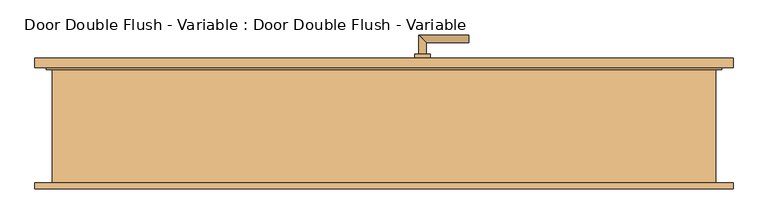
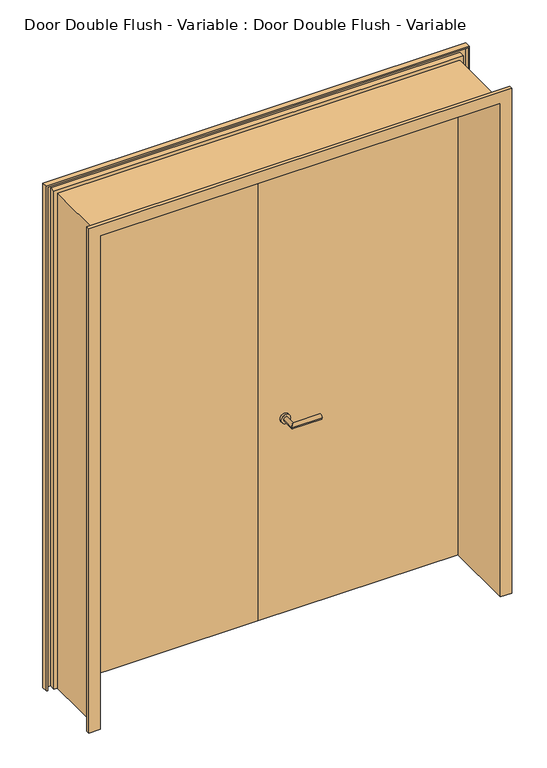
"""IFC4 building model written with IfcOpenShell, lengths in millimetres: door geometry, Door Double Flush - Variable : Door Double Flush - Variable."""

from ifc_helpers import new_model, si_unit, point, frame, frame_2d, origin, place, context, project, spatial, polyline, circle_curve, ellipse_curve, trimmed, segment, composite_curve, outline, extrude, faceted_brep, source, transform, mapped, element, save
from ifc_brep_helpers import plane_surface, cylinder_surface, advanced_brep


def door_double_flush_variable_door_double_flush_variable_ac6c3b87(model_context):
    return source(origin(), model_context, "Body", "SolidModel", [
        advanced_brep(
        [(90.0, 139.4346141, 1000.0), (110.0, 139.4346141, 1000.0), (90.0, 69.4346141, 1000.0), (110.0, 89.4346141, 1000.0), (220.0, 69.4346141, 1000.0), (220.0, 89.4346141, 1000.0)],
        [
            (0, 1, circle_curve(frame((100.0, 139.4346141, 1000.0), z_axis=(0.0, 1.0, 0.0), x_axis=(1.0, 0.0, 0.0)), 10.0)),
            (1, 0, circle_curve(frame((100.0, 139.4346141, 1000.0), z_axis=(0.0, 1.0, 0.0), x_axis=(1.0, 0.0, 0.0)), 10.0)),
            (0, 2),
            (2, 3, ellipse_curve(frame((100.0, 79.4346141, 1000.0), z_axis=(-0.7071067811865385, 0.7071067811865565, 0.0), x_axis=(0.7071067811865563, 0.7071067811865386, 0.0)), 14.1421356, 10.0)),
            (3, 1),
            (3, 2, ellipse_curve(frame((100.0, 79.4346141, 1000.0), z_axis=(-0.7071067811865385, 0.7071067811865565, 0.0), x_axis=(0.7071067811865563, 0.7071067811865386, 0.0)), 14.1421356, 10.0)),
            (4, 5, circle_curve(frame((220.0, 79.4346141, 1000.0), z_axis=(1.0, 0.0, 0.0), x_axis=(0.0, 1.0, 0.0)), 10.0)),
            (5, 4, circle_curve(frame((220.0, 79.4346141, 1000.0), z_axis=(1.0, 0.0, 0.0), x_axis=(0.0, 1.0, 0.0)), 10.0)),
            (2, 4),
            (5, 3),
        ],
        [
            plane_surface(frame((100.0, 139.4346141, -287.7526403), z_axis=(0.0, 1.0, 0.0), x_axis=(0.0, 0.0, 1.0))),
            cylinder_surface(frame((100.0, 139.4346141, 1000.0), z_axis=(0.0, 1.0, 0.0), x_axis=(1.0, 0.0, 0.0)), 10.0),
            plane_surface(frame((220.0, 79.4346141, -287.7526403), z_axis=(1.0, 0.0, 0.0), x_axis=(0.0, 0.0, 1.0))),
            cylinder_surface(frame((100.0, 79.4346141, 1000.0), z_axis=(-1.0, 0.0, 0.0), x_axis=(0.0, 1.0, 0.0)), 10.0),
        ],
        [
            (0, [[1, 2]]),
            (1, [[-1, 3, 4, 5]]),
            (1, [[-2, -5, 6, -3]]),
            (2, [[7, 8]]),
            (3, [[-4, 9, -8, 10]]),
            (3, [[-6, -10, -7, -9]]),
        ],
    ),
        advanced_brep(
        [(110.0, 199.4346141, 1000.0), (90.0, 199.4346141, 1000.0), (110.0, 229.4346141, 1000.0), (90.0, 249.4346141, 1000.0), (220.0, 229.4346141, 1000.0), (220.0, 249.4346141, 1000.0)],
        [
            (0, 1, circle_curve(frame((100.0, 199.4346141, 1000.0), z_axis=(0.0, -1.0, 0.0), x_axis=(-1.0, 0.0, 0.0)), 10.0)),
            (1, 0, circle_curve(frame((100.0, 199.4346141, 1000.0), z_axis=(0.0, -1.0, 0.0), x_axis=(-1.0, 0.0, 0.0)), 10.0)),
            (0, 2),
            (2, 3, ellipse_curve(frame((100.0, 239.4346141, 1000.0), z_axis=(-0.7071067811865475, -0.7071067811865475, 0.0), x_axis=(0.7071067811865474, -0.7071067811865476, 0.0)), 14.1421356, 10.0)),
            (3, 1),
            (3, 2, ellipse_curve(frame((100.0, 239.4346141, 1000.0), z_axis=(-0.7071067811865475, -0.7071067811865475, 0.0), x_axis=(0.7071067811865474, -0.7071067811865476, 0.0)), 14.1421356, 10.0)),
            (4, 5, circle_curve(frame((220.0, 239.4346141, 1000.0), z_axis=(1.0, 0.0, 0.0), x_axis=(0.0, 1.0, 0.0)), 10.0)),
            (5, 4, circle_curve(frame((220.0, 239.4346141, 1000.0), z_axis=(1.0, 0.0, 0.0), x_axis=(0.0, 1.0, 0.0)), 10.0)),
            (2, 4),
            (5, 3),
        ],
        [
            plane_surface(frame((100.0, 199.4346141, -287.7526403), z_axis=(0.0, -1.0, 0.0), x_axis=(0.0, 0.0, 1.0))),
            cylinder_surface(frame((100.0, 199.4346141, 1000.0), z_axis=(0.0, -1.0, 0.0), x_axis=(-1.0, 0.0, 0.0)), 10.0),
            plane_surface(frame((220.0, 239.4346141, -287.7526403), z_axis=(1.0, 0.0, 0.0), x_axis=(0.0, 0.0, 1.0))),
            cylinder_surface(frame((100.0, 239.4346141, 1000.0), z_axis=(-1.0, 0.0, 0.0), x_axis=(0.0, 1.0, 0.0)), 10.0),
        ],
        [
            (0, [[1, 2]]),
            (1, [[-1, 3, 4, 5]]),
            (1, [[-2, -5, 6, -3]]),
            (2, [[7, 8]]),
            (3, [[-4, 9, -8, 10]]),
            (3, [[-6, -10, -7, -9]]),
        ],
    ),
        extrude(outline(composite_curve([segment(trimmed(circle_curve(frame_2d((1000.0, 100.0)), 20.0), [point((1000.0, 80.0))], [point((1000.0, 120.0))], False, "CARTESIAN"), True, "CONTINUOUS"), segment(trimmed(circle_curve(frame_2d((1000.0, 100.0)), 20.0), [point((1000.0, 120.0))], [point((1000.0, 80.0))], False, "CARTESIAN"), True, "CONTINUOUS")], self_intersect=False)), frame((0.0, 129.4346141, 0.0), z_axis=(0.0, 1.0, 0.0), x_axis=(0.0, 0.0, 1.0)), (0.0, 0.0, 1.0), 10.0),
        extrude(outline(composite_curve([segment(trimmed(circle_curve(frame_2d((1000.0, 100.0)), 20.0), [point((1000.0, 80.0))], [point((1000.0, 120.0))], False, "CARTESIAN"), True, "CONTINUOUS"), segment(trimmed(circle_curve(frame_2d((1000.0, 100.0)), 20.0), [point((1000.0, 120.0))], [point((1000.0, 80.0))], False, "CARTESIAN"), True, "CONTINUOUS")], self_intersect=False)), frame((0.0, 189.4346141, 0.0), z_axis=(0.0, 1.0, 0.0), x_axis=(0.0, 0.0, 1.0)), (0.0, 0.0, 1.0), 10.0),
        extrude(outline(polyline([(0.0, 164.4346141), (-871.25, 164.4346141), (-871.25, 189.4346141), (0.0, 189.4346141), (0.0, 164.4346141)])), frame((0.0, 0.0, 100.0), z_axis=(0.0, 0.0, 1.0), x_axis=(1.0, 0.0, 0.0)), (0.0, 0.0, 1.0), 2250.0),
        extrude(outline(polyline([(871.25, 164.4346141), (0.0, 164.4346141), (0.0, 189.4346141), (871.25, 189.4346141), (871.25, 164.4346141)])), frame((0.0, 0.0, 100.0), z_axis=(0.0, 0.0, 1.0), x_axis=(1.0, 0.0, 0.0)), (0.0, 0.0, 1.0), 2250.0),
        faceted_brep([(905.75, -150.5653859, 100.0), (856.25, -150.5653859, 100.0), (856.25, 164.4346141, 100.0), (871.25, 164.4346141, 100.0), (871.25, 189.4346141, 100.0), (905.75, 189.4346141, 100.0), (905.75, 164.4346141, 100.0), (900.75, 164.4346141, 100.0), (900.75, 184.4346141, 100.0), (876.25, 184.4346141, 100.0), (876.25, 159.4346141, 100.0), (861.25, 159.4346141, 100.0), (861.25, -145.5653859, 100.0), (900.75, -145.5653859, 100.0), (900.75, -135.5653859, 100.0), (905.75, -135.5653859, 100.0), (905.75, -150.5653859, 2384.5), (-905.75, -150.5653859, 2384.5), (-905.75, -150.5653859, 100.0), (-856.25, -150.5653859, 100.0), (-856.25, -150.5653859, 2335.0), (856.25, -150.5653859, 2335.0), (856.25, 164.4346141, 2335.0), (-856.25, 164.4346141, 2335.0), (-856.25, 164.4346141, 100.0), (-871.25, 164.4346141, 100.0), (-871.25, 164.4346141, 2350.0), (871.25, 164.4346141, 2350.0), (871.25, 189.4346141, 2350.0), (-871.25, 189.4346141, 2350.0), (-871.25, 189.4346141, 100.0), (-905.75, 189.4346141, 100.0), (-905.75, 189.4346141, 2384.5), (905.75, 189.4346141, 2384.5), (905.75, 164.4346141, 2384.5), (-905.75, 164.4346141, 2384.5), (-905.75, 164.4346141, 100.0), (-900.75, 164.4346141, 100.0), (-900.75, 164.4346141, 2379.5), (900.75, 164.4346141, 2379.5), (900.75, 184.4346141, 2379.5), (-900.75, 184.4346141, 2379.5), (-900.75, 184.4346141, 100.0), (-876.25, 184.4346141, 100.0), (-876.25, 184.4346141, 2355.0), (876.25, 184.4346141, 2355.0), (876.25, 159.4346141, 2355.0), (-876.25, 159.4346141, 2355.0), (-876.25, 159.4346141, 100.0), (-861.25, 159.4346141, 100.0), (-861.25, 159.4346141, 2340.0), (861.25, 159.4346141, 2340.0), (861.25, -145.5653859, 2340.0), (-861.25, -145.5653859, 2340.0), (-861.25, -145.5653859, 100.0), (-900.75, -145.5653859, 100.0), (-900.75, -145.5653859, 2379.5), (900.75, -145.5653859, 2379.5), (900.75, -135.5653859, 2379.5), (-900.75, -135.5653859, 2379.5), (-900.75, -135.5653859, 100.0), (-905.75, -135.5653859, 100.0), (-905.75, -135.5653859, 2384.5), (905.75, -135.5653859, 2384.5)], [[[0, 1, 2, 3, 4, 5, 6, 7, 8, 9, 10, 11, 12, 13, 14, 15]], [[1, 0, 16, 17, 18, 19, 20, 21]], [[2, 1, 21, 22]], [[3, 2, 22, 23, 24, 25, 26, 27]], [[4, 3, 27, 28]], [[5, 4, 28, 29, 30, 31, 32, 33]], [[6, 5, 33, 34]], [[7, 6, 34, 35, 36, 37, 38, 39]], [[8, 7, 39, 40]], [[9, 8, 40, 41, 42, 43, 44, 45]], [[10, 9, 45, 46]], [[11, 10, 46, 47, 48, 49, 50, 51]], [[12, 11, 51, 52]], [[13, 12, 52, 53, 54, 55, 56, 57]], [[14, 13, 57, 58]], [[15, 14, 58, 59, 60, 61, 62, 63]], [[0, 15, 63, 16]], [[17, 62, 61, 18]], [[18, 61, 60, 55, 54, 49, 48, 43, 42, 37, 36, 31, 30, 25, 24, 19]], [[23, 20, 19, 24]], [[29, 26, 25, 30]], [[35, 32, 31, 36]], [[41, 38, 37, 42]], [[47, 44, 43, 48]], [[53, 50, 49, 54]], [[59, 56, 55, 60]], [[22, 21, 20, 23]], [[28, 27, 26, 29]], [[34, 33, 32, 35]], [[40, 39, 38, 41]], [[46, 45, 44, 47]], [[52, 51, 50, 53]], [[58, 57, 56, 59]], [[16, 63, 62, 17]]]),
    ])


if __name__ == "__main__":
    model = new_model("IFC4")
    model_context = context("Model", 3, world=origin())
    ifc_project = project(units=[si_unit("LENGTHUNIT", "METRE", prefix="MILLI")], contexts=[model_context])
    site = spatial("IfcSite", under=ifc_project)
    building = spatial("IfcBuilding", under=site)
    placement = place(None, origin())
    door_double_flush_variable_door_double_flush_variable_shape = door_double_flush_variable_door_double_flush_variable_ac6c3b87(model_context)
    element("IfcDoor", 1, ObjectType="Door Double Flush - Variable : Door Double Flush - Variable", at=placement, inside=building, context=model_context, shape_type="MappedRepresentation", body=[
        mapped(door_double_flush_variable_door_double_flush_variable_shape, transform((0.0, 0.0, 0.0), x_axis=(1.0, 0.0, 0.0), y_axis=(0.0, 1.0, 0.0), z_axis=(0.0, 0.0, 1.0))),
    ])
    save(model, "model.ifc")

# Revit data of these elements
# Type "Door Double Flush - Variable : Door Double Flush - Variable"
#   Type Mark = "33"
#   Operation = "DoubleDoorSingleSwing"
#   Keynote = "16.03"
#   Rough Width [instance default] = 2.010 m
#   Rough Height [instance default] = 2.360 m
#   Doorhandle Height = 0.900 m
#   Height [instance default] = 2.260 m
#   Sill Height [instance default] = 0.100 m
#   Width [instance default] = 2.010 m
#   Visibility [instance default] = yes
#   Doorhandle choose [instance default] = element 138974
#   Doorhandle [instance default] = Metal _ Chrome
#   Door [instance default] = Door - Wood
#   Frame [instance default] = Door - Wood
#   Function = (empty or 0)
#   Wall Closure = (empty or 0)
#   Assembly Code = ""
# Element 1 (IfcDoor, "Door Double Flush - Variable : Door Double Flush - Variable")
#   Rough Width = 1.7625 m
#   Width = 1.7625 m
#   Materials on its faces: "Door - Wood", "Metal _ Chrome"
# Materials
#   "Metal _ Chrome": class "Metall", colour RGB 247 247 247, transparency 0
#   "Door - Wood": class "Unassigned", colour RGB 114 94 79, transparency 0
